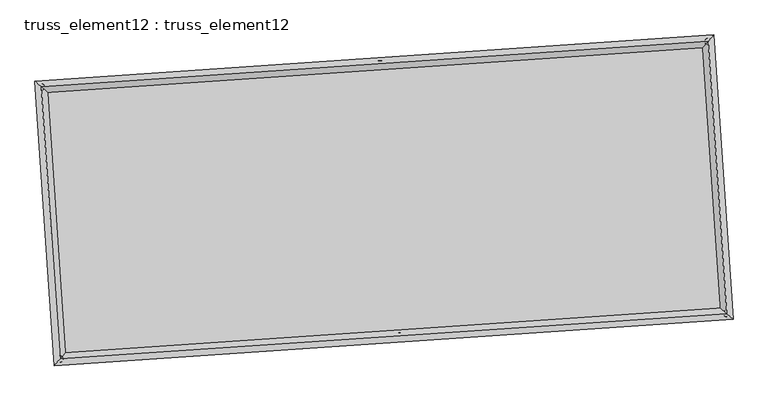
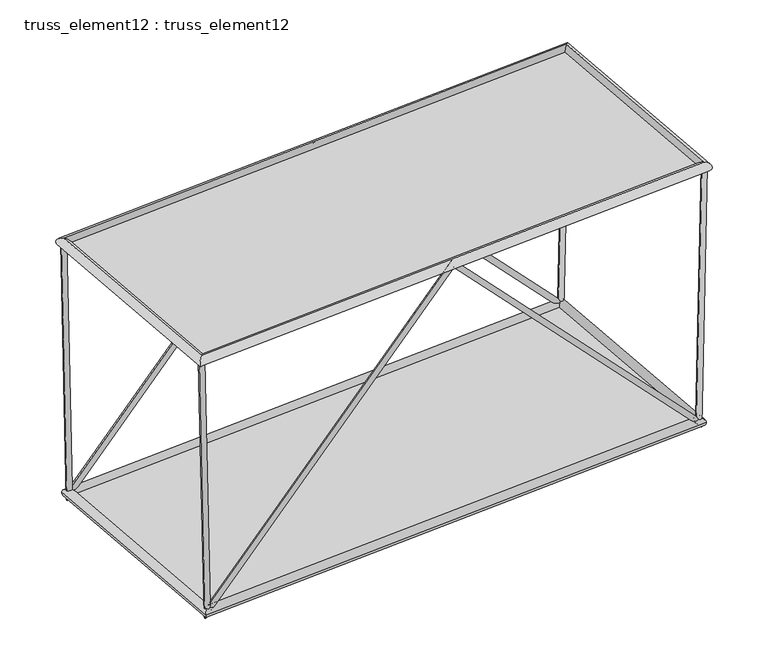
"""IFC4 building model written with IfcOpenShell, lengths in millimetres: plate geometry, truss_element12 : truss_element12."""

from ifc_helpers import new_model, si_unit, frame, origin, origin_with_axes, place, context, project, spatial, polyline, circle_curve, ellipse_curve, outline, extrude, source, transform, mapped, element, save
from ifc_brep_helpers import plane_surface, cylinder_surface, advanced_brep


def truss_element12_truss_element12_086eec47(model_context):
    return source(origin(), model_context, "Body", "SolidModel", [
        advanced_brep(
        [(-3774.2332872, 2268.7717745, 4999.8930544), (-3873.3127666, 2255.4121866, 4997.7071475), (-3667.5840303, 2276.0437819, 121.4126505), (-3761.4028525, 2263.0428982, -121.4126505), (1064.2299582, 2598.6881905, 5070.9037686), (1064.6705353, 2592.1144969, 4926.674072), (5795.0471287, 2921.2646298, 121.4057099), (5889.7138483, 2921.1158587, -121.4057099), (5902.6858035, 2928.6041019, 4999.8808289), (6002.6612371, 2928.8173118, 4997.6746502)],
        [
            (0, 1, circle_curve(frame((-3823.7730269, 2262.0919805, 4998.800101), z_axis=(-0.021855917096439963, -0.0014902719046873062, 0.9997600201936082), x_axis=(-0.13359639491826203, 0.9910347724122863, -0.0014433068183134015)), 50.0)),
            (1, 0, circle_curve(frame((-3823.7730269, 2262.0919805, 4998.800101), z_axis=(-0.021855917096439963, -0.0014902719046873062, 0.9997600201936082), x_axis=(-0.13359639491826203, 0.9910347724122863, -0.0014433068183134015)), 50.0)),
            (0, 2),
            (2, 3, ellipse_curve(frame((-3714.4934414, 2269.54334, 0.0), z_axis=(-0.9297759208968324, -0.06339788563679134, 0.3626257644145429), x_axis=(0.3617857041453493, 0.024668791889457715, 0.9319348448162931)), 130.5638727, 50.0)),
            (3, 1),
            (3, 2, ellipse_curve(frame((-3714.4934414, 2269.54334, 0.0), z_axis=(-0.9297759208968324, -0.06339788563679134, 0.3626257644145429), x_axis=(0.3617857041453493, 0.024668791889457715, 0.9319348448162931)), 130.5638727, 50.0)),
            (2, 4),
            (4, 5, ellipse_curve(frame((1064.4502467, 2595.4013437, 4998.7889203), z_axis=(-0.9976833946750359, -0.06802823813325232, 5.297341116267986e-05), x_axis=(-5.285069275020394e-05, -3.6036878343152564e-06, -0.9999999985969089)), 72.2718761, 50.0)),
            (5, 3),
            (5, 4, ellipse_curve(frame((1064.4502467, 2595.4013437, 4998.7889203), z_axis=(-0.9976833946750359, -0.06802823813325232, 5.297341116267986e-05), x_axis=(-5.285069275020394e-05, -3.6036878343152564e-06, -0.9999999985969089)), 72.2718761, 50.0)),
            (4, 6),
            (6, 7, ellipse_curve(frame((5842.3804885, 2921.1902443, 0.0), z_axis=(-0.9298318338903021, -0.06340169813127101, -0.36248170348069864), x_axis=(-0.3616419769436296, -0.024658991677930685, 0.9319908876387853)), 130.5485583, 50.0)),
            (7, 5),
            (7, 6, ellipse_curve(frame((5842.3804885, 2921.1902443, 0.0), z_axis=(-0.9298318338903021, -0.06340169813127101, -0.36248170348069864), x_axis=(-0.3616419769436296, -0.024658991677930685, 0.9319908876387853)), 130.5485583, 50.0)),
            (8, 9, circle_curve(frame((5952.6735203, 2928.7107068, 4998.7777396), z_axis=(0.022058606365204667, 0.0015040925154303942, 0.9997555479170547), x_axis=(-0.002164760807071468, 0.9999965959239133, -0.00145669188023135)), 50.0)),
            (9, 8, circle_curve(frame((5952.6735203, 2928.7107068, 4998.7777396), z_axis=(0.022058606365204667, 0.0015040925154303942, 0.9997555479170547), x_axis=(-0.002164760807071468, 0.9999965959239133, -0.00145669188023135)), 50.0)),
            (6, 8),
            (9, 7),
        ],
        [
            plane_surface(frame((-3823.7730269, 2312.091925, 4998.8746324), z_axis=(-0.021855917096441312, -0.0014902719046848139, 0.9997600201936081), x_axis=(0.9997611309147169, -3.257904132603074e-05, 0.02185589281481271))),
            cylinder_surface(frame((-3823.7730269, 2262.0919805, 4998.800101), z_axis=(-0.021855917096439963, -0.0014902719046873062, 0.9997600201936082), x_axis=(-0.13359639491826203, 0.9910347724122863, -0.0014433068183134015)), 50.0),
            cylinder_surface(frame((-3714.4934414, 2269.54334, 0.0), z_axis=(-0.6902675071609972, -0.0470667173608615, -0.7220218090020663), x_axis=(-0.020420682259035285, 0.9987517940373583, -0.04558343606217084)), 50.0),
            cylinder_surface(frame((1064.4502467, 2595.4013437, 4998.7889203), z_axis=(-0.6901911845814975, -0.04706151321429475, 0.7220951064091002), x_axis=(-0.11534499746176513, 0.9922792658247876, -0.045578395921375275)), 50.0),
            plane_surface(frame((5952.6735203, 2878.7107634, 4998.8529625), z_axis=(0.022058606365203737, 0.0015040925154315723, 0.9997555479170548), x_axis=(0.9997566793401409, -3.318625963721899e-05, -0.022058581401513063))),
            cylinder_surface(frame((5842.3804885, 2921.1902443, 0.0), z_axis=(-0.022058606365204667, -0.0015040925154303942, -0.9997555479170547), x_axis=(-0.002164760807071468, 0.9999965959239133, -0.00145669188023135)), 50.0),
        ],
        [
            (0, [[1, 2]]),
            (1, [[-1, 3, 4, 5]]),
            (1, [[-2, -5, 6, -3]]),
            (2, [[-4, 7, 8, 9]]),
            (2, [[-6, -9, 10, -7]]),
            (3, [[-8, 11, 12, 13]]),
            (3, [[-10, -13, 14, -11]]),
            (4, [[15, 16]]),
            (5, [[-12, 17, -16, 18]]),
            (5, [[-14, -18, -15, -17]]),
        ],
    ),
        advanced_brep(
        [(-3502.1203343, -1721.9618098, 4999.8930544), (-3601.1998136, -1735.3213977, 4997.7071475), (-3395.4710774, -1714.6898024, 121.4126505), (-3489.2898996, -1727.6906861, -121.4126505), (1336.3429111, -1392.0453938, 5070.9037686), (1336.7834882, -1398.6190874, 4926.674072), (6067.1600816, -1069.4689545, 121.4057099), (6161.8268012, -1069.6177256, -121.4057099), (6174.7987565, -1062.1294824, 4999.8808289), (6274.77419, -1061.9162725, 4997.6746502)],
        [
            (0, 1, circle_curve(frame((-3551.660074, -1728.6416038, 4998.800101), z_axis=(-0.02185591709644024, -0.001490271904687352, 0.9997600201936082), x_axis=(-0.13359639491826175, 0.9910347724122863, -0.0014433068183133876)), 50.0)),
            (1, 0, circle_curve(frame((-3551.660074, -1728.6416038, 4998.800101), z_axis=(-0.02185591709644024, -0.001490271904687352, 0.9997600201936082), x_axis=(-0.13359639491826175, 0.9910347724122863, -0.0014433068183133876)), 50.0)),
            (0, 2),
            (2, 3, ellipse_curve(frame((-3442.3804885, -1721.1902443, 0.0), z_axis=(-0.9297759208968323, -0.06339788563679132, 0.36262576441454303), x_axis=(0.3617857041453494, 0.024668791889457687, 0.9319348448162932)), 130.5638727, 50.0)),
            (3, 1),
            (3, 2, ellipse_curve(frame((-3442.3804885, -1721.1902443, 0.0), z_axis=(-0.9297759208968323, -0.06339788563679132, 0.36262576441454303), x_axis=(0.3617857041453494, 0.024668791889457687, 0.9319348448162932)), 130.5638727, 50.0)),
            (2, 4),
            (4, 5, ellipse_curve(frame((1336.5631996, -1395.3322406, 4998.7889203), z_axis=(-0.9976833946750359, -0.06802823813325233, 5.2973411162840336e-05), x_axis=(-5.285069275035771e-05, -3.6036878342575984e-06, -0.9999999985969089)), 72.2718761, 50.0)),
            (5, 3),
            (5, 4, ellipse_curve(frame((1336.5631996, -1395.3322406, 4998.7889203), z_axis=(-0.9976833946750359, -0.06802823813325233, 5.2973411162840336e-05), x_axis=(-5.285069275035771e-05, -3.6036878342575984e-06, -0.9999999985969089)), 72.2718761, 50.0)),
            (4, 6),
            (6, 7, ellipse_curve(frame((6114.4934414, -1069.54334, 0.0), z_axis=(-0.9298318338903019, -0.06340169813127097, -0.3624817034806985), x_axis=(-0.3616419769436298, -0.024658991677930772, 0.9319908876387852)), 130.5485583, 50.0)),
            (7, 5),
            (7, 6, ellipse_curve(frame((6114.4934414, -1069.54334, 0.0), z_axis=(-0.9298318338903019, -0.06340169813127097, -0.3624817034806985), x_axis=(-0.3616419769436298, -0.024658991677930772, 0.9319908876387852)), 130.5485583, 50.0)),
            (8, 9, circle_curve(frame((6224.7864732, -1062.0228775, 4998.7777396), z_axis=(0.022058606365204722, 0.0015040925154303226, 0.9997555479170547), x_axis=(-0.0021647608070713776, 0.9999965959239133, -0.0014566918802312804)), 50.0)),
            (9, 8, circle_curve(frame((6224.7864732, -1062.0228775, 4998.7777396), z_axis=(0.022058606365204722, 0.0015040925154303226, 0.9997555479170547), x_axis=(-0.0021647608070713776, 0.9999965959239133, -0.0014566918802312804)), 50.0)),
            (6, 8),
            (9, 7),
        ],
        [
            plane_surface(frame((-3551.660074, -1678.6416593, 4998.8746324), z_axis=(-0.021855917096441312, -0.0014902719046848097, 0.9997600201936081), x_axis=(0.9997611309147169, -3.257904132603074e-05, 0.02185589281481271))),
            cylinder_surface(frame((-3551.660074, -1728.6416038, 4998.800101), z_axis=(-0.02185591709644024, -0.001490271904687352, 0.9997600201936082), x_axis=(-0.13359639491826175, 0.9910347724122863, -0.0014433068183133876)), 50.0),
            cylinder_surface(frame((-3442.3804885, -1721.1902443, 0.0), z_axis=(-0.6902675071609972, -0.04706671736086146, -0.722021809002066), x_axis=(-0.02042068225903536, 0.9987517940373583, -0.04558343606217072)), 50.0),
            cylinder_surface(frame((1336.5631996, -1395.3322406, 4998.7889203), z_axis=(-0.6901911845814976, -0.04706151321429482, 0.7220951064091004), x_axis=(-0.11534499746176505, 0.9922792658247878, -0.04557839592137508)), 50.0),
            plane_surface(frame((6224.7864732, -1112.0228209, 4998.8529625), z_axis=(0.022058606365203737, 0.0015040925154315703, 0.9997555479170548), x_axis=(0.9997566793401409, -3.318625963721899e-05, -0.022058581401513063))),
            cylinder_surface(frame((6114.4934414, -1069.54334, 0.0), z_axis=(-0.022058606365204722, -0.0015040925154303226, -0.9997555479170547), x_axis=(-0.0021647608070713776, 0.9999965959239133, -0.0014566918802312804)), 50.0),
        ],
        [
            (0, [[1, 2]]),
            (1, [[-1, 3, 4, 5]]),
            (1, [[-2, -5, 6, -3]]),
            (2, [[-4, 7, 8, 9]]),
            (2, [[-6, -9, 10, -7]]),
            (3, [[-8, 11, 12, 13]]),
            (3, [[-10, -13, 14, -11]]),
            (4, [[15, 16]]),
            (5, [[-12, 17, -16, 18]]),
            (5, [[-14, -18, -15, -17]]),
        ],
    ),
        advanced_brep(
        [(-3551.6658856, -1728.6480451, 4908.8001012), (-3551.6542623, -1728.6351625, 5088.8001008), (-3823.7663947, 2262.0863877, 5088.8001008), (-3823.7796591, 2262.0975733, 4908.8001012), (5952.6681185, 2928.7042935, 5088.7777394), (5952.6789222, 2928.7171202, 4908.7777398), (6224.7802508, -1062.0172567, 5088.7777394), (6224.7926957, -1062.0284982, 4908.7777398)],
        [
            (0, 1, ellipse_curve(frame((-3551.660074, -1728.6416038, 4998.800101), z_axis=(-0.7535719234036229, 0.6573654662782041, 1.6135980928572344e-06), x_axis=(-0.6573654662762421, -0.7535719234053343, 1.6135980928572024e-06)), 127.2792206, 90.0)),
            (1, 2),
            (2, 3, ellipse_curve(frame((-3823.7730269, 2262.0919805, 4998.800101), z_axis=(-0.6573654662762419, -0.7535719234053345, 1.61359809285717e-06), x_axis=(0.7535719234036229, -0.6573654662782039, -1.6135980928572026e-06)), 127.2792206, 90.0)),
            (3, 0),
            (1, 0, ellipse_curve(frame((-3551.660074, -1728.6416038, 4998.800101), z_axis=(-0.7535719234036229, 0.6573654662782041, 1.6135980928572344e-06), x_axis=(-0.6573654662762421, -0.7535719234053343, 1.6135980928572024e-06)), 127.2792206, 90.0)),
            (3, 2, ellipse_curve(frame((-3823.7730269, 2262.0919805, 4998.800101), z_axis=(-0.6573654662762419, -0.7535719234053345, 1.61359809285717e-06), x_axis=(0.7535719234036229, -0.6573654662782039, -1.6135980928572026e-06)), 127.2792206, 90.0)),
            (2, 4),
            (4, 5, ellipse_curve(frame((5952.6735203, 2928.7107068, 4998.7777396), z_axis=(-0.7535719234036229, 0.657365466278204, 1.6135980928571717e-06), x_axis=(-0.657365466276242, -0.7535719234053344, 1.6135980928572015e-06)), 127.2792206, 90.0)),
            (5, 3),
            (5, 4, ellipse_curve(frame((5952.6735203, 2928.7107068, 4998.7777396), z_axis=(-0.7535719234036229, 0.657365466278204, 1.6135980928571717e-06), x_axis=(-0.657365466276242, -0.7535719234053344, 1.6135980928572015e-06)), 127.2792206, 90.0)),
            (4, 6),
            (6, 7, ellipse_curve(frame((6224.7864732, -1062.0228775, 4998.7777396), z_axis=(0.657365466276242, 0.7535719234053344, -1.6135980928572333e-06), x_axis=(-0.7535719234036229, 0.6573654662782041, 1.6135980928572032e-06)), 127.2792206, 90.0)),
            (7, 5),
            (7, 6, ellipse_curve(frame((6224.7864732, -1062.0228775, 4998.7777396), z_axis=(0.657365466276242, 0.7535719234053344, -1.6135980928572333e-06), x_axis=(-0.7535719234036229, 0.6573654662782041, 1.6135980928572032e-06)), 127.2792206, 90.0)),
            (6, 1),
            (0, 7),
        ],
        [
            cylinder_surface(frame((-3551.660074, -1728.6416038, 4998.800101), z_axis=(0.06802823822870424, -0.9976833960748764, 0.0), x_axis=(-0.9976833936796619, -0.06802823806538366, 6.929323559275387e-05)), 90.0),
            cylinder_surface(frame((-3823.7730269, 2262.0919805, 4998.800101), z_axis=(-0.997683396072279, -0.06802823822852651, 2.2819723071379943e-06), x_axis=(-0.0680282379233993, 0.997683393845226, 6.701126329073946e-05)), 90.0),
            cylinder_surface(frame((5952.6735203, 2928.7107068, 4998.7777396), z_axis=(-0.06802823822870425, 0.9976833960748764, 0.0), x_axis=(0.997683393984789, 0.06802823808618913, 6.472929098872504e-05)), 90.0),
            cylinder_surface(frame((6224.7864732, -1062.0228775, 4998.7777396), z_axis=(0.9976833960722788, 0.06802823822852633, -2.2819723071380388e-06), x_axis=(0.06802823822852633, -0.9976833938244204, 6.701126329073944e-05)), 90.0),
        ],
        [
            (0, [[1, 2, 3, 4]]),
            (0, [[5, -4, 6, -2]]),
            (1, [[-3, 7, 8, 9]]),
            (1, [[-6, -9, 10, -7]]),
            (2, [[-8, 11, 12, 13]]),
            (2, [[-10, -13, 14, -11]]),
            (3, [[-12, 15, -1, 16]]),
            (3, [[-14, -16, -5, -15]]),
        ],
    ),
        advanced_brep(
        [(-3358.7115243, -1625.2761972, 0.0), (-3526.0494527, -1817.1042913, 0.0), (-3810.4074885, 2353.2123043, 0.0), (-3618.5793943, 2185.8743758, 0.0), (5926.0494527, 3017.1042913, 0.0), (5758.7115243, 2825.2761972, 0.0), (6210.4074885, -1153.2123043, 0.0), (6018.5793943, -985.8743758, 0.0)],
        [
            (0, 1, ellipse_curve(frame((-3442.3804885, -1721.1902443, 0.0), z_axis=(-0.7535719234054589, 0.6573654662780798, 0.0), x_axis=(-0.6573654662780798, -0.7535719234054589, 0.0)), 127.2792206, 90.0)),
            (1, 2),
            (2, 3, ellipse_curve(frame((-3714.4934414, 2269.54334, 0.0), z_axis=(-0.6573654662780798, -0.7535719234054589, 0.0), x_axis=(0.7535719234054589, -0.6573654662780799, 0.0)), 127.2792206, 90.0)),
            (3, 0),
            (1, 0, ellipse_curve(frame((-3442.3804885, -1721.1902443, 0.0), z_axis=(-0.7535719234054589, 0.6573654662780798, 0.0), x_axis=(-0.6573654662780798, -0.7535719234054589, 0.0)), 127.2792206, 90.0)),
            (3, 2, ellipse_curve(frame((-3714.4934414, 2269.54334, 0.0), z_axis=(-0.6573654662780798, -0.7535719234054589, 0.0), x_axis=(0.7535719234054589, -0.6573654662780799, 0.0)), 127.2792206, 90.0)),
            (2, 4),
            (4, 5, ellipse_curve(frame((5842.3804885, 2921.1902443, 0.0), z_axis=(-0.7535719234054589, 0.6573654662780798, 0.0), x_axis=(-0.6573654662780797, -0.753571923405459, 0.0)), 127.2792206, 90.0)),
            (5, 3),
            (5, 4, ellipse_curve(frame((5842.3804885, 2921.1902443, 0.0), z_axis=(-0.7535719234054589, 0.6573654662780798, 0.0), x_axis=(-0.6573654662780797, -0.753571923405459, 0.0)), 127.2792206, 90.0)),
            (4, 6),
            (6, 7, ellipse_curve(frame((6114.4934414, -1069.54334, 0.0), z_axis=(0.6573654662780798, 0.7535719234054589, 0.0), x_axis=(-0.753571923405459, 0.6573654662780797, 0.0)), 127.2792206, 90.0)),
            (7, 5),
            (7, 6, ellipse_curve(frame((6114.4934414, -1069.54334, 0.0), z_axis=(0.6573654662780798, 0.7535719234054589, 0.0), x_axis=(-0.753571923405459, 0.6573654662780797, 0.0)), 127.2792206, 90.0)),
            (6, 1),
            (0, 7),
        ],
        [
            cylinder_surface(frame((-3442.3804885, -1721.1902443, 0.0), z_axis=(0.06802823822870296, -0.9976833960748764, 0.0), x_axis=(-0.9976833960748764, -0.06802823822870296, 0.0)), 90.0),
            cylinder_surface(frame((-3714.4934414, 2269.54334, 0.0), z_axis=(-0.9976833960748765, -0.06802823822870219, 0.0), x_axis=(-0.06802823822870219, 0.9976833960748765, 0.0)), 90.0),
            cylinder_surface(frame((5842.3804885, 2921.1902443, 0.0), z_axis=(-0.06802823822870291, 0.9976833960748764, 0.0), x_axis=(0.9976833960748764, 0.06802823822870291, 0.0)), 90.0),
            cylinder_surface(frame((6114.4934414, -1069.54334, 0.0), z_axis=(0.9976833960748765, 0.06802823822870213, 0.0), x_axis=(0.06802823822870213, -0.9976833960748765, 0.0)), 90.0),
        ],
        [
            (0, [[1, 2, 3, 4]]),
            (0, [[5, -4, 6, -2]]),
            (1, [[-3, 7, 8, 9]]),
            (1, [[-6, -9, 10, -7]]),
            (2, [[-8, 11, 12, 13]]),
            (2, [[-10, -13, 14, -11]]),
            (3, [[-12, 15, -1, 16]]),
            (3, [[-14, -16, -5, -15]]),
        ],
    ),
        extrude(outline(polyline([(-3442.3804885, -1721.1902443), (-3714.4934414, 2269.54334), (5842.3804885, 2921.1902443), (6114.4934414, -1069.54334), (-3442.3804885, -1721.1902443)])), origin_with_axes(), (0.0, 0.0, 1.0), 20.0),
        extrude(outline(polyline([(-2000.0, 4899.5736452), (2000.0, 4899.5736452), (2000.0, -4899.5736451), (-2000.0, -4899.5736451), (-2000.0, 4899.5736452)])), frame((1200.5067232, 600.0345515, 4998.7889203), z_axis=(2.2766858811342764e-06, 1.5523855574128772e-07, 0.9999999999973964), x_axis=(-0.06802823822870292, 0.9976833960748765, 0.0)), (0.0, 0.0, 1.0), 20.0),
    ])


if __name__ == "__main__":
    model = new_model("IFC4")
    model_context = context("Model", 3, world=origin())
    ifc_project = project(units=[si_unit("LENGTHUNIT", "METRE", prefix="MILLI")], contexts=[model_context])
    site = spatial("IfcSite", under=ifc_project)
    building = spatial("IfcBuilding", under=site)
    placement = place(None, origin())
    truss_element12_truss_element12_shape = truss_element12_truss_element12_086eec47(model_context)
    element("IfcPlate", 1, ObjectType="truss_element12 : truss_element12", at=placement, inside=building, context=model_context, shape_type="MappedRepresentation", body=[
        mapped(truss_element12_truss_element12_shape, transform((0.0, 0.0, 0.0), x_axis=(1.0, 0.0, 0.0), y_axis=(0.0, 1.0, 0.0), z_axis=(0.0, 0.0, 1.0))),
    ])
    save(model, "model.ifc")

# Revit data of these elements
# Type "truss_element12 : truss_element12"
#   steellbar1 = 90 mm
#   steelbar2 = 50 mm
#   offset1 = 5000 mm
#   M = Default Roof
# Element 1 (IfcPlate, "truss_element12 : truss_element12")
#   Materials on its faces: "Default Roof"
# Materials
#   "Default Roof": class "Miscellaneous", colour RGB 0 127 0, transparency 0, Comments = "Rendering appearance not upgraded Rendering appearance not upgraded ", Cost = 0
